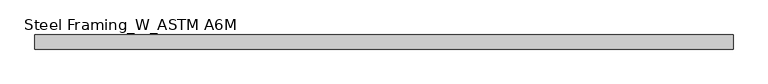
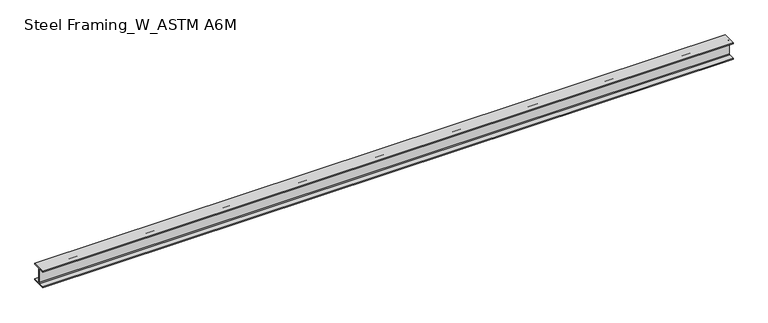
"""IFC4 building model written with IfcOpenShell, lengths in millimetres: beam geometry, Steel Framing_W_ASTM A6M : H_SB_AR_S02_W250x49.1_RB3."""

from ifc_helpers import new_model, si_unit, point, frame, frame_2d, origin, place, context, project, spatial, polyline, circle_curve, trimmed, segment, composite_curve, outline, extrude, source, transform, mapped, element, save


def steel_framing_w_astm_a6m_6b1bb185(model_context):
    return source(origin(), model_context, "Body", "SweptSolid", [
        extrude(outline(composite_curve([segment(polyline([(101.0, -112.5), (101.0, -123.5), (-101.0, -123.5), (-101.0, -112.5), (-16.385, -112.5)]), True, "CONTINUOUS"), segment(trimmed(circle_curve(frame_2d((-16.385, -99.8)), 12.7), [point((-16.385, -112.5))], [point((-3.685, -99.8))], True, "CARTESIAN"), True, "CONTINUOUS"), segment(polyline([(-3.685, -99.8), (-3.685, 99.8)]), True, "CONTINUOUS"), segment(trimmed(circle_curve(frame_2d((-16.385, 99.8)), 12.7), [point((-3.685, 99.8))], [point((-16.385, 112.5))], True, "CARTESIAN"), True, "CONTINUOUS"), segment(polyline([(-16.385, 112.5), (-101.0, 112.5), (-101.0, 123.5), (101.0, 123.5), (101.0, 112.5), (16.385, 112.5)]), True, "CONTINUOUS"), segment(trimmed(circle_curve(frame_2d((16.385, 99.8)), 12.7), [point((16.385, 112.5))], [point((3.685, 99.8))], True, "CARTESIAN"), True, "CONTINUOUS"), segment(polyline([(3.685, 99.8), (3.685, -99.8)]), True, "CONTINUOUS"), segment(trimmed(circle_curve(frame_2d((16.385, -99.8)), 12.7), [point((3.685, -99.8))], [point((16.385, -112.5))], True, "CARTESIAN"), True, "CONTINUOUS"), segment(polyline([(16.385, -112.5), (101.0, -112.5)]), True, "CONTINUOUS")], self_intersect=False)), frame((-4987.2, 0.0, 0.0), z_axis=(1.0, 0.0, 0.0), x_axis=(0.0, 1.0, 0.0)), (0.0, 0.0, 1.0), 9987.2),
    ])


if __name__ == "__main__":
    model = new_model("IFC4")
    model_context = context("Model", 3, world=origin())
    ifc_project = project(units=[si_unit("LENGTHUNIT", "METRE", prefix="MILLI")], contexts=[model_context])
    site = spatial("IfcSite", under=ifc_project)
    building = spatial("IfcBuilding", under=site)
    placement = place(None, origin())
    steel_framing_w_astm_a6m_shape = steel_framing_w_astm_a6m_6b1bb185(model_context)
    element("IfcBeam", 1, ObjectType="Steel Framing_W_ASTM A6M : H_SB_AR_S02_W250x49.1_RB3", at=placement, inside=building, context=model_context, shape_type="MappedRepresentation", body=[
        mapped(steel_framing_w_astm_a6m_shape, transform((0.0, 0.0, 0.0), x_axis=(1.0, 0.0, 0.0), y_axis=(0.0, 1.0, 0.0), z_axis=(0.0, 0.0, 1.0))),
    ])
    save(model, "model.ifc")

# Revit data of these elements
# Type "Steel Framing_W_ASTM A6M : H_SB_AR_S02_W250x49.1_RB3"
#   Type Mark = "RB3"
#   Section Name Key = "W10x33"
#   Width = 20.2 cm
#   Web Thickness = 0.737 cm
#   Web Fillet = 1.27 cm
#   Warping Constant = 212000.0 cm⁶
#   Torsional Moment of Inertia = 24.30 cm⁴
#   Section Area = 62.6 cm²
#   Plastic Modulus weak axis = 229.0 cm³
#   Plastic Modulus strong axis = 636.0 cm³
#   Perimeter = 1.27 m²/m
#   Nominal Weight = 49.10 kgf/m
#   Moment of Inertia weak axis = 1520.00 cm⁴
#   Moment of Inertia strong axis = 7120.00 cm⁴
#   Height = 24.7 cm
#   Flange Thickness = 1.1 cm
#   Elastic Modulus weak axis = 151.0 cm³
#   Elastic Modulus strong axis = 574.0 cm³
#   Centroid Vertical = 12.35 cm
#   Centroid Horizontal = 10.1 cm
#   Length [instance default] = 1500 mm
#   Structural Material [instance default] = Steel, 45-345
#   Bolt Spacing = 0
#   Assembly Code = ""
# Element 1 (IfcBeam, "Steel Framing_W_ASTM A6M : H_SB_AR_S02_W250x49.1_RB3")
#   Materials on its faces: "Steel, 45-345"
# Materials
#   "Steel, 45-345": class "Metal", colour RGB 189 187 185, transparency 0, Description = "Steel 345 MPa", Cost = 0
